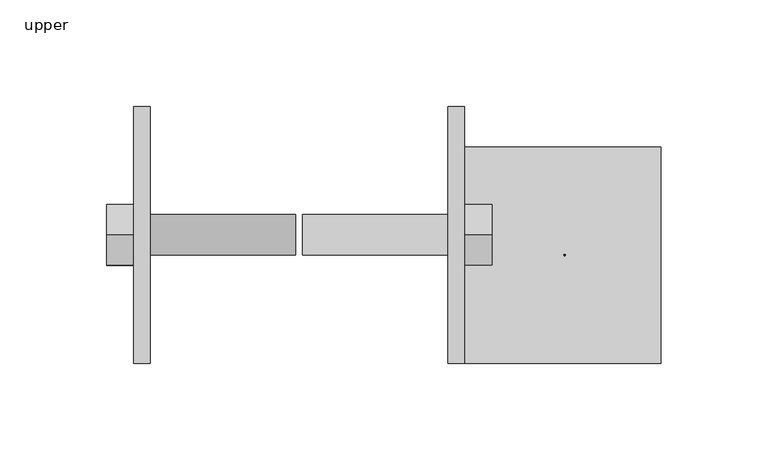
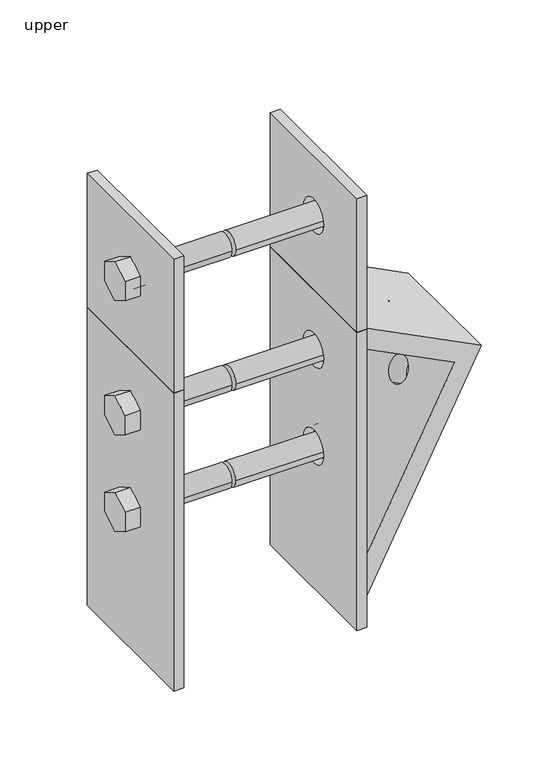
"""IFC4 building model written with IfcOpenShell, lengths in millimetres: fastener geometry, 060523 - W_P_C - Fastenings - Column Base & Top with X Bracing - Custom : upper."""

from ifc_helpers import new_model, si_unit, point, frame, frame_2d, origin, place, context, project, spatial, polyline, circle_curve, trimmed, segment, composite_curve, outline, extrude, source, transform, mapped, element, save
from ifc_brep_helpers import plane_surface, revolved_surface, advanced_brep


def upper_50ad7738(model_context):
    return source(origin(), model_context, "Body", "SolidModel", [
        advanced_brep(
        [(-77.7875, 60.325, 261.9375), (-77.7875, -52.3875, 261.9375), (-77.7875, -60.325, 261.9375), (-69.85, -60.325, 261.9375), (-69.85, 60.325, 261.9375), (-77.7875, 60.325, 7.9375), (-77.7875, -52.3875, 7.9375), (-77.7875, -60.325, 7.9375), (-77.7875, -13.890625, 211.1375), (-77.7875, 13.890625, 211.1375), (-77.7875, -13.890625, 128.5875), (-77.7875, 13.890625, 128.5875), (-69.85, 60.325, 7.9375), (-69.85, -60.325, 7.9375), (-69.85, 13.890625, 211.1375), (-69.85, -13.890625, 211.1375), (-69.85, 13.890625, 128.5875), (-69.85, -13.890625, 128.5875)],
        [
            (0, 1),
            (1, 2),
            (2, 3),
            (3, 4),
            (4, 0),
            (0, 5),
            (5, 6),
            (6, 7),
            (7, 2),
            (8, 9, circle_curve(frame((-77.7875, 0.0, 211.1375), z_axis=(1.0, 0.0, 0.0), x_axis=(0.0, -1.0, 0.0)), 13.890625)),
            (9, 8, circle_curve(frame((-77.7875, 0.0, 211.1375), z_axis=(1.0, 0.0, 0.0), x_axis=(0.0, -1.0, 0.0)), 13.890625)),
            (10, 11, circle_curve(frame((-77.7875, 0.0, 128.5875), z_axis=(1.0, 0.0, 0.0), x_axis=(0.0, -1.0, 0.0)), 13.890625)),
            (11, 10, circle_curve(frame((-77.7875, 0.0, 128.5875), z_axis=(1.0, 0.0, 0.0), x_axis=(0.0, -1.0, 0.0)), 13.890625)),
            (4, 12),
            (12, 5),
            (7, 13),
            (13, 3),
            (14, 9),
            (8, 15),
            (15, 14, circle_curve(frame((-69.85, 0.0, 211.1375), z_axis=(1.0, 0.0, 0.0), x_axis=(0.0, -1.0, 0.0)), 13.890625)),
            (14, 15, circle_curve(frame((-69.85, 0.0, 211.1375), z_axis=(1.0, 0.0, 0.0), x_axis=(0.0, -1.0, 0.0)), 13.890625)),
            (16, 11),
            (10, 17),
            (17, 16, circle_curve(frame((-69.85, 0.0, 128.5875), z_axis=(1.0, 0.0, 0.0), x_axis=(0.0, -1.0, 0.0)), 13.890625)),
            (16, 17, circle_curve(frame((-69.85, 0.0, 128.5875), z_axis=(1.0, 0.0, 0.0), x_axis=(0.0, -1.0, 0.0)), 13.890625)),
            (13, 12),
        ],
        [
            plane_surface(frame((-77.7875, -60.325, 261.9375), z_axis=(0.0, 0.0, 1.0), x_axis=(1.0, 0.0, 0.0))),
            plane_surface(frame((-77.7875, 60.325, 261.9375), z_axis=(-1.0, 0.0, 0.0), x_axis=(0.0, 1.0, 0.0))),
            plane_surface(frame((-77.7875, 60.325, 261.9375), z_axis=(0.0, 1.0, 0.0), x_axis=(1.0, 0.0, 0.0))),
            plane_surface(frame((-77.7875, -60.325, 7.9375), z_axis=(0.0, -1.0, 0.0), x_axis=(1.0, 0.0, 0.0))),
            revolved_surface(polyline([(-77.7875, -13.890625, 211.1375), (-69.85, -13.890625, 211.1375)]), (-69.85, 0.0, 211.1375), (-1.0, 0.0, 0.0)),
            revolved_surface(polyline([(-77.7875, -13.890625, 128.5875), (-69.85, -13.890625, 128.5875)]), (-69.85, 0.0, 128.5875), (-1.0, 0.0, 0.0)),
            plane_surface(frame((-69.85, 60.325, 261.9375), z_axis=(1.0, 0.0, 0.0), x_axis=(0.0, -1.0, 0.0))),
            plane_surface(frame((-77.7875, 60.325, 7.9375), z_axis=(0.0, 0.0, -1.0), x_axis=(1.0, 0.0, 0.0))),
        ],
        [
            (0, [[1, 2, 3, 4, 5]]),
            (1, [[-2, -1, 6, 7, 8, 9], [10, 11], [12, 13]]),
            (2, [[-6, -5, 14, 15]]),
            (3, [[-9, 16, 17, -3]]),
            (4, [[18, -10, 19, 20]]),
            (4, [[-18, 21, -19, -11]]),
            (5, [[22, -12, 23, 24]]),
            (5, [[-22, 25, -23, -13]]),
            (6, [[-17, 26, -14, -4], [-20, -21], [-24, -25]]),
            (7, [[-8, -7, -15, -26, -16]]),
        ],
    ),
        extrude(outline(polyline([(14.2875, 219.386392), (14.2875, 202.888608), (0.0, 194.6397161), (-14.2875, 202.888608), (-14.2875, 219.386392), (0.0, 227.6352839), (14.2875, 219.386392)])), frame((-90.4875, 0.0, 0.0), z_axis=(1.0, 0.0, 0.0), x_axis=(0.0, 1.0, 0.0)), (0.0, 0.0, 1.0), 12.7),
        extrude(outline(composite_curve([segment(trimmed(circle_curve(frame_2d((0.0, 211.1375)), 9.525), [point((9.525, 211.1375))], [point((-9.525, 211.1375))], False, "CARTESIAN"), True, "CONTINUOUS"), segment(trimmed(circle_curve(frame_2d((0.0, 211.1375)), 9.525), [point((-9.525, 211.1375))], [point((9.525, 211.1375))], False, "CARTESIAN"), True, "CONTINUOUS")], self_intersect=False)), frame((-77.7875, 0.0, 0.0), z_axis=(1.0, 0.0, 0.0), x_axis=(0.0, 1.0, 0.0)), (0.0, 0.0, 1.0), 76.2),
        extrude(outline(polyline([(14.2875, 136.836392), (14.2875, 120.338608), (0.0, 112.0897161), (-14.2875, 120.338608), (-14.2875, 136.836392), (0.0, 145.0852839), (14.2875, 136.836392)])), frame((-90.4875, 0.0, 0.0), z_axis=(1.0, 0.0, 0.0), x_axis=(0.0, 1.0, 0.0)), (0.0, 0.0, 1.0), 12.7),
        extrude(outline(composite_curve([segment(trimmed(circle_curve(frame_2d((0.0, 128.5875)), 9.525), [point((9.525, 128.5875))], [point((-9.525, 128.5875))], False, "CARTESIAN"), True, "CONTINUOUS"), segment(trimmed(circle_curve(frame_2d((0.0, 128.5875)), 9.525), [point((-9.525, 128.5875))], [point((9.525, 128.5875))], False, "CARTESIAN"), True, "CONTINUOUS")], self_intersect=False)), frame((-77.7875, 0.0, 0.0), z_axis=(1.0, 0.0, 0.0), x_axis=(0.0, 1.0, 0.0)), (0.0, 0.0, 1.0), 76.2),
        extrude(outline(polyline([(14.2875, 219.386392), (14.2875, 202.888608), (0.0, 194.6397161), (-14.2875, 202.888608), (-14.2875, 219.386392), (0.0, 227.6352839), (14.2875, 219.386392)])), frame((-90.4875, 0.0, 0.0), z_axis=(1.0, 0.0, 0.0), x_axis=(0.0, 1.0, 0.0)), (0.0, 0.0, 1.0), 12.7),
        extrude(outline(composite_curve([segment(trimmed(circle_curve(frame_2d((0.0, 211.1375)), 9.525), [point((9.525, 211.1375))], [point((-9.525, 211.1375))], False, "CARTESIAN"), True, "CONTINUOUS"), segment(trimmed(circle_curve(frame_2d((0.0, 211.1375)), 9.525), [point((-9.525, 211.1375))], [point((9.525, 211.1375))], False, "CARTESIAN"), True, "CONTINUOUS")], self_intersect=False)), frame((-77.7875, 0.0, 0.0), z_axis=(1.0, 0.0, 0.0), x_axis=(0.0, 1.0, 0.0)), (0.0, 0.0, 1.0), 76.2),
        advanced_brep(
        [(77.7875, 60.325, 261.9375), (69.85, 60.325, 261.9375), (69.85, -60.325, 261.9375), (77.7875, -60.325, 261.9375), (77.7875, -52.3875, 261.9375), (77.7875, -60.325, 7.9375), (77.7875, -52.3875, 7.9375), (77.7875, 60.325, 7.9375), (77.7875, -13.890625, 211.1375), (77.7875, 13.890625, 211.1375), (77.7875, -13.890625, 128.5875), (77.7875, 13.890625, 128.5875), (69.85, 60.325, 7.9375), (69.85, -60.325, 7.9375), (69.85, 13.890625, 211.1375), (69.85, -13.890625, 211.1375), (69.85, 13.890625, 128.5875), (69.85, -13.890625, 128.5875)],
        [
            (0, 1),
            (1, 2),
            (2, 3),
            (3, 4),
            (4, 0),
            (3, 5),
            (5, 6),
            (6, 7),
            (7, 0),
            (8, 9, circle_curve(frame((77.7875, 0.0, 211.1375), z_axis=(-1.0, 0.0, 0.0), x_axis=(0.0, -1.0, 0.0)), 13.890625)),
            (9, 8, circle_curve(frame((77.7875, 0.0, 211.1375), z_axis=(-1.0, 0.0, 0.0), x_axis=(0.0, -1.0, 0.0)), 13.890625)),
            (10, 11, circle_curve(frame((77.7875, 0.0, 128.5875), z_axis=(-1.0, 0.0, 0.0), x_axis=(0.0, -1.0, 0.0)), 13.890625)),
            (11, 10, circle_curve(frame((77.7875, 0.0, 128.5875), z_axis=(-1.0, 0.0, 0.0), x_axis=(0.0, -1.0, 0.0)), 13.890625)),
            (7, 12),
            (12, 1),
            (2, 13),
            (13, 5),
            (14, 15, circle_curve(frame((69.85, 0.0, 211.1375), z_axis=(-1.0, 0.0, 0.0), x_axis=(0.0, -1.0, 0.0)), 13.890625)),
            (15, 8),
            (9, 14),
            (15, 14, circle_curve(frame((69.85, 0.0, 211.1375), z_axis=(-1.0, 0.0, 0.0), x_axis=(0.0, -1.0, 0.0)), 13.890625)),
            (16, 17, circle_curve(frame((69.85, 0.0, 128.5875), z_axis=(-1.0, 0.0, 0.0), x_axis=(0.0, -1.0, 0.0)), 13.890625)),
            (17, 10),
            (11, 16),
            (17, 16, circle_curve(frame((69.85, 0.0, 128.5875), z_axis=(-1.0, 0.0, 0.0), x_axis=(0.0, -1.0, 0.0)), 13.890625)),
            (12, 13),
        ],
        [
            plane_surface(frame((77.7875, -60.325, 261.9375), z_axis=(0.0, 0.0, 1.0), x_axis=(-1.0, 0.0, 0.0))),
            plane_surface(frame((77.7875, 60.325, 261.9375), z_axis=(1.0, 0.0, 0.0), x_axis=(0.0, 1.0, 0.0))),
            plane_surface(frame((77.7875, 60.325, 261.9375), z_axis=(0.0, 1.0, 0.0), x_axis=(-1.0, 0.0, 0.0))),
            plane_surface(frame((77.7875, -60.325, 7.9375), z_axis=(0.0, -1.0, 0.0), x_axis=(-1.0, 0.0, 0.0))),
            revolved_surface(polyline([(77.7875, -13.890625, 211.1375), (69.85, -13.890625, 211.1375)]), (69.85, 0.0, 211.1375), (1.0, 0.0, 0.0)),
            revolved_surface(polyline([(77.7875, -13.890625, 128.5875), (69.85, -13.890625, 128.5875)]), (69.85, 0.0, 128.5875), (1.0, 0.0, 0.0)),
            plane_surface(frame((69.85, 60.325, 261.9375), z_axis=(-1.0, 0.0, 0.0), x_axis=(0.0, -1.0, 0.0))),
            plane_surface(frame((77.7875, 60.325, 7.9375), z_axis=(0.0, 0.0, -1.0), x_axis=(-1.0, 0.0, 0.0))),
        ],
        [
            (0, [[1, 2, 3, 4, 5]]),
            (1, [[6, 7, 8, 9, -5, -4], [10, 11], [12, 13]]),
            (2, [[14, 15, -1, -9]]),
            (3, [[-3, 16, 17, -6]]),
            (4, [[18, 19, -11, 20]]),
            (4, [[-10, -19, 21, -20]]),
            (5, [[22, 23, -13, 24]]),
            (5, [[-12, -23, 25, -24]]),
            (6, [[-2, -15, 26, -16], [-21, -18], [-25, -22]]),
            (7, [[-17, -26, -14, -8, -7]]),
        ],
    ),
        extrude(outline(polyline([(14.2875, 219.386392), (14.2875, 202.888608), (0.0, 194.6397161), (-14.2875, 202.888608), (-14.2875, 219.386392), (0.0, 227.6352839), (14.2875, 219.386392)])), frame((77.7875, 0.0, 0.0), z_axis=(1.0, 0.0, 0.0), x_axis=(0.0, 1.0, 0.0)), (0.0, 0.0, 1.0), 12.7),
        extrude(outline(composite_curve([segment(trimmed(circle_curve(frame_2d((0.0, 211.1375)), 9.525), [point((9.525, 211.1375))], [point((-9.525, 211.1375))], False, "CARTESIAN"), True, "CONTINUOUS"), segment(trimmed(circle_curve(frame_2d((0.0, 211.1375)), 9.525), [point((-9.525, 211.1375))], [point((9.525, 211.1375))], False, "CARTESIAN"), True, "CONTINUOUS")], self_intersect=False)), frame((1.5875, 0.0, 0.0), z_axis=(1.0, 0.0, 0.0), x_axis=(0.0, 1.0, 0.0)), (0.0, 0.0, 1.0), 76.2),
        extrude(outline(polyline([(14.2875, 136.836392), (14.2875, 120.338608), (0.0, 112.0897161), (-14.2875, 120.338608), (-14.2875, 136.836392), (0.0, 145.0852839), (14.2875, 136.836392)])), frame((77.7875, 0.0, 0.0), z_axis=(1.0, 0.0, 0.0), x_axis=(0.0, 1.0, 0.0)), (0.0, 0.0, 1.0), 12.7),
        extrude(outline(composite_curve([segment(trimmed(circle_curve(frame_2d((0.0, 128.5875)), 9.525), [point((9.525, 128.5875))], [point((-9.525, 128.5875))], False, "CARTESIAN"), True, "CONTINUOUS"), segment(trimmed(circle_curve(frame_2d((0.0, 128.5875)), 9.525), [point((-9.525, 128.5875))], [point((9.525, 128.5875))], False, "CARTESIAN"), True, "CONTINUOUS")], self_intersect=False)), frame((1.5875, 0.0, 0.0), z_axis=(1.0, 0.0, 0.0), x_axis=(0.0, 1.0, 0.0)), (0.0, 0.0, 1.0), 76.2),
        extrude(outline(polyline([(14.2875, 219.386392), (14.2875, 202.888608), (0.0, 194.6397161), (-14.2875, 202.888608), (-14.2875, 219.386392), (0.0, 227.6352839), (14.2875, 219.386392)])), frame((77.7875, 0.0, 0.0), z_axis=(1.0, 0.0, 0.0), x_axis=(0.0, 1.0, 0.0)), (0.0, 0.0, 1.0), 12.7),
        extrude(outline(composite_curve([segment(trimmed(circle_curve(frame_2d((0.0, 211.1375)), 9.525), [point((9.525, 211.1375))], [point((-9.525, 211.1375))], False, "CARTESIAN"), True, "CONTINUOUS"), segment(trimmed(circle_curve(frame_2d((0.0, 211.1375)), 9.525), [point((-9.525, 211.1375))], [point((9.525, 211.1375))], False, "CARTESIAN"), True, "CONTINUOUS")], self_intersect=False)), frame((1.5875, 0.0, 0.0), z_axis=(1.0, 0.0, 0.0), x_axis=(0.0, 1.0, 0.0)), (0.0, 0.0, 1.0), 76.2),
        advanced_brep(
        [(-77.7875, -60.325, 376.2375), (-77.7875, 60.325, 376.2375), (-77.7875, 60.325, 261.9375), (-77.7875, 52.3875, 261.9375), (-77.7875, -60.325, 261.9375), (-77.7875, -13.890625, 325.4375), (-77.7875, 13.890625, 325.4375), (-69.85, -60.325, 376.2375), (-69.85, 60.325, 376.2375), (-69.85, 60.325, 261.9375), (-69.85, -60.325, 261.9375), (-69.85, 13.890625, 325.4375), (-69.85, -13.890625, 325.4375)],
        [
            (0, 1),
            (1, 2),
            (2, 3),
            (3, 4),
            (4, 0),
            (5, 6, circle_curve(frame((-77.7875, 0.0, 325.4375), z_axis=(1.0, 0.0, 0.0), x_axis=(0.0, -1.0, 0.0)), 13.890625)),
            (6, 5, circle_curve(frame((-77.7875, 0.0, 325.4375), z_axis=(1.0, 0.0, 0.0), x_axis=(0.0, -1.0, 0.0)), 13.890625)),
            (0, 7),
            (7, 8),
            (8, 1),
            (8, 9),
            (9, 2),
            (4, 10),
            (10, 7),
            (11, 6),
            (5, 12),
            (12, 11, circle_curve(frame((-69.85, 0.0, 325.4375), z_axis=(1.0, 0.0, 0.0), x_axis=(0.0, -1.0, 0.0)), 13.890625)),
            (11, 12, circle_curve(frame((-69.85, 0.0, 325.4375), z_axis=(1.0, 0.0, 0.0), x_axis=(0.0, -1.0, 0.0)), 13.890625)),
            (10, 9),
        ],
        [
            plane_surface(frame((-77.7875, 60.325, 376.2375), z_axis=(-1.0, 0.0, 0.0), x_axis=(0.0, 1.0, 0.0))),
            plane_surface(frame((-77.7875, -60.325, 376.2375), z_axis=(0.0, 0.0, 1.0), x_axis=(1.0, 0.0, 0.0))),
            plane_surface(frame((-77.7875, 60.325, 376.2375), z_axis=(0.0, 1.0, 0.0), x_axis=(1.0, 0.0, 0.0))),
            plane_surface(frame((-77.7875, -60.325, 261.9375), z_axis=(0.0, -1.0, 0.0), x_axis=(1.0, 0.0, 0.0))),
            revolved_surface(polyline([(-77.7875, -13.890625, 325.4375), (-69.85, -13.890625, 325.4375)]), (-69.85, 0.0, 325.4375), (-1.0, 0.0, 0.0)),
            plane_surface(frame((-69.85, 60.325, 376.2375), z_axis=(1.0, 0.0, 0.0), x_axis=(0.0, -1.0, 0.0))),
            plane_surface(frame((-77.7875, 60.325, 261.9375), z_axis=(0.0, 0.0, -1.0), x_axis=(1.0, 0.0, 0.0))),
        ],
        [
            (0, [[1, 2, 3, 4, 5], [6, 7]]),
            (1, [[-1, 8, 9, 10]]),
            (2, [[-2, -10, 11, 12]]),
            (3, [[-5, 13, 14, -8]]),
            (4, [[15, -6, 16, 17]]),
            (4, [[-15, 18, -16, -7]]),
            (5, [[-14, 19, -11, -9], [-17, -18]]),
            (6, [[-4, -3, -12, -19, -13]]),
        ],
    ),
        extrude(outline(polyline([(14.2875, 333.686392), (14.2875, 317.188608), (0.0, 308.9397161), (-14.2875, 317.188608), (-14.2875, 333.686392), (0.0, 341.9352839), (14.2875, 333.686392)])), frame((-90.4875, 0.0, 0.0), z_axis=(1.0, 0.0, 0.0), x_axis=(0.0, 1.0, 0.0)), (0.0, 0.0, 1.0), 12.7),
        extrude(outline(composite_curve([segment(trimmed(circle_curve(frame_2d((0.0, 325.4375)), 9.525), [point((9.525, 325.4375))], [point((-9.525, 325.4375))], False, "CARTESIAN"), True, "CONTINUOUS"), segment(trimmed(circle_curve(frame_2d((0.0, 325.4375)), 9.525), [point((-9.525, 325.4375))], [point((9.525, 325.4375))], False, "CARTESIAN"), True, "CONTINUOUS")], self_intersect=False)), frame((-77.7875, 0.0, 0.0), z_axis=(1.0, 0.0, 0.0), x_axis=(0.0, 1.0, 0.0)), (0.0, 0.0, 1.0), 76.2),
        advanced_brep(
        [(77.7875, -60.325, 376.2375), (77.7875, -60.325, 261.9375), (77.7875, 52.3875, 261.9375), (77.7875, 60.325, 261.9375), (77.7875, 60.325, 376.2375), (77.7875, -13.890625, 325.4375), (77.7875, 13.890625, 325.4375), (69.85, 60.325, 376.2375), (69.85, -60.325, 376.2375), (69.85, 60.325, 261.9375), (69.85, -60.325, 261.9375), (69.85, 13.890625, 325.4375), (69.85, -13.890625, 325.4375)],
        [
            (0, 1),
            (1, 2),
            (2, 3),
            (3, 4),
            (4, 0),
            (5, 6, circle_curve(frame((77.7875, 0.0, 325.4375), z_axis=(-1.0, 0.0, 0.0), x_axis=(0.0, -1.0, 0.0)), 13.890625)),
            (6, 5, circle_curve(frame((77.7875, 0.0, 325.4375), z_axis=(-1.0, 0.0, 0.0), x_axis=(0.0, -1.0, 0.0)), 13.890625)),
            (4, 7),
            (7, 8),
            (8, 0),
            (3, 9),
            (9, 7),
            (8, 10),
            (10, 1),
            (11, 12, circle_curve(frame((69.85, 0.0, 325.4375), z_axis=(-1.0, 0.0, 0.0), x_axis=(0.0, -1.0, 0.0)), 13.890625)),
            (12, 5),
            (6, 11),
            (12, 11, circle_curve(frame((69.85, 0.0, 325.4375), z_axis=(-1.0, 0.0, 0.0), x_axis=(0.0, -1.0, 0.0)), 13.890625)),
            (9, 10),
        ],
        [
            plane_surface(frame((77.7875, 60.325, 376.2375), z_axis=(1.0, 0.0, 0.0), x_axis=(0.0, 1.0, 0.0))),
            plane_surface(frame((77.7875, -60.325, 376.2375), z_axis=(0.0, 0.0, 1.0), x_axis=(-1.0, 0.0, 0.0))),
            plane_surface(frame((77.7875, 60.325, 376.2375), z_axis=(0.0, 1.0, 0.0), x_axis=(-1.0, 0.0, 0.0))),
            plane_surface(frame((77.7875, -60.325, 261.9375), z_axis=(0.0, -1.0, 0.0), x_axis=(-1.0, 0.0, 0.0))),
            revolved_surface(polyline([(77.7875, -13.890625, 325.4375), (69.85, -13.890625, 325.4375)]), (69.85, 0.0, 325.4375), (1.0, 0.0, 0.0)),
            plane_surface(frame((69.85, 60.325, 376.2375), z_axis=(-1.0, 0.0, 0.0), x_axis=(0.0, -1.0, 0.0))),
            plane_surface(frame((77.7875, 60.325, 261.9375), z_axis=(0.0, 0.0, -1.0), x_axis=(-1.0, 0.0, 0.0))),
        ],
        [
            (0, [[1, 2, 3, 4, 5], [6, 7]]),
            (1, [[8, 9, 10, -5]]),
            (2, [[11, 12, -8, -4]]),
            (3, [[-10, 13, 14, -1]]),
            (4, [[15, 16, -7, 17]]),
            (4, [[-6, -16, 18, -17]]),
            (5, [[-9, -12, 19, -13], [-18, -15]]),
            (6, [[-14, -19, -11, -3, -2]]),
        ],
    ),
        extrude(outline(polyline([(14.2875, 333.686392), (14.2875, 317.188608), (0.0, 308.9397161), (-14.2875, 317.188608), (-14.2875, 333.686392), (0.0, 341.9352839), (14.2875, 333.686392)])), frame((77.7875, 0.0, 0.0), z_axis=(1.0, 0.0, 0.0), x_axis=(0.0, 1.0, 0.0)), (0.0, 0.0, 1.0), 12.7),
        extrude(outline(composite_curve([segment(trimmed(circle_curve(frame_2d((0.0, 325.4375)), 9.525), [point((9.525, 325.4375))], [point((-9.525, 325.4375))], False, "CARTESIAN"), True, "CONTINUOUS"), segment(trimmed(circle_curve(frame_2d((0.0, 325.4375)), 9.525), [point((-9.525, 325.4375))], [point((9.525, 325.4375))], False, "CARTESIAN"), True, "CONTINUOUS")], self_intersect=False)), frame((1.5875, 0.0, 0.0), z_axis=(1.0, 0.0, 0.0), x_axis=(0.0, 1.0, 0.0)), (0.0, 0.0, 1.0), 76.2),
        advanced_brep(
        [(170.0383695, 41.275, 215.9775257), (77.7875, 41.275, 34.925), (77.7875, 41.275, 69.8926921), (148.6865418, 41.275, 209.0398963), (77.7875, 41.275, 245.1647625), (77.7875, 41.275, 262.9816915), (170.0383695, -60.325, 215.9775257), (77.7875, -60.325, 262.9816915), (77.7875, -60.325, 245.1647625), (148.6865418, -60.325, 209.0398963), (77.7875, -60.325, 69.8926921), (77.7875, -60.325, 34.925), (125.1288563, -9.525, 238.8600656), (124.4216199, -9.525, 239.2204206), (117.2145207, -9.525, 225.075692), (117.9217571, -9.525, 224.7153371), (137.6957155, -9.525, 187.4691853), (127.9661316, -9.525, 168.3738017), (142.1108602, -9.525, 161.1667025), (151.8404441, -9.525, 180.2620861)],
        [
            (0, 1),
            (1, 2),
            (2, 3),
            (3, 4),
            (4, 5),
            (5, 0),
            (6, 7),
            (7, 8),
            (8, 9),
            (9, 10),
            (10, 11),
            (11, 6),
            (5, 7),
            (6, 0),
            (12, 13, circle_curve(frame((124.7752381, -9.525, 239.0402431), z_axis=(-0.45399049973954897, 0.0, -0.8910065241883668), x_axis=(-0.8910065241883668, 0.0, 0.45399049973954897)), 0.396875)),
            (13, 12, circle_curve(frame((124.7752381, -9.525, 239.0402431), z_axis=(-0.45399049973954897, 0.0, -0.8910065241883668), x_axis=(-0.8910065241883668, 0.0, 0.45399049973954897)), 0.396875)),
            (4, 8),
            (3, 9),
            (14, 15, circle_curve(frame((117.5681389, -9.525, 224.8955145), z_axis=(0.45399049973954897, 0.0, 0.8910065241883668), x_axis=(-0.8910065241883668, 0.0, 0.45399049973954897)), 0.396875)),
            (15, 14, circle_curve(frame((117.5681389, -9.525, 224.8955145), z_axis=(0.45399049973954897, 0.0, 0.8910065241883668), x_axis=(-0.8910065241883668, 0.0, 0.45399049973954897)), 0.396875)),
            (2, 10),
            (16, 17, circle_curve(frame((132.8309236, -9.525, 177.9214935), z_axis=(0.8910065241883661, 0.0, -0.4539904997395502), x_axis=(0.4539904997395502, 0.0, 0.8910065241883661)), 10.715625)),
            (17, 16, circle_curve(frame((132.8309236, -9.525, 177.9214935), z_axis=(0.8910065241883661, 0.0, -0.4539904997395502), x_axis=(0.4539904997395502, 0.0, 0.8910065241883661)), 10.715625)),
            (1, 11),
            (18, 19, circle_curve(frame((146.9756522, -9.525, 170.7143943), z_axis=(-0.8910065241883661, 0.0, 0.4539904997395502), x_axis=(0.4539904997395502, 0.0, 0.8910065241883661)), 10.715625)),
            (19, 18, circle_curve(frame((146.9756522, -9.525, 170.7143943), z_axis=(-0.8910065241883661, 0.0, 0.4539904997395502), x_axis=(0.4539904997395502, 0.0, 0.8910065241883661)), 10.715625)),
            (13, 14),
            (15, 12),
            (19, 16),
            (17, 18),
        ],
        [
            plane_surface(frame((77.7875, 41.275, 262.9816915), z_axis=(0.0, 1.0, 0.0), x_axis=(-0.8910065241883668, 0.0, 0.45399049973954897))),
            plane_surface(frame((77.7875, -60.325, 262.9816915), z_axis=(0.0, -1.0, 0.0), x_axis=(0.8910065241883668, 0.0, -0.45399049973954897))),
            plane_surface(frame((170.0383695, 41.275, 215.9775257), z_axis=(0.45399049973954897, 0.0, 0.8910065241883668), x_axis=(0.0, -1.0, 0.0))),
            plane_surface(frame((77.7875, 41.275, 262.9816915), z_axis=(-1.0, 0.0, 0.0), x_axis=(0.0, -1.0, 0.0))),
            plane_surface(frame((77.7875, 41.275, 245.1647625), z_axis=(-0.4539904997395488, 0.0, -0.8910065241883668), x_axis=(0.0, -1.0, 0.0))),
            plane_surface(frame((148.6865418, 41.275, 209.0398963), z_axis=(-0.8910065241883659, 0.0, 0.45399049973955063), x_axis=(0.0, -1.0, 0.0))),
            plane_surface(frame((77.7875, 41.275, 69.8926921), z_axis=(-1.0, 0.0, 0.0), x_axis=(0.0, -1.0, 0.0))),
            plane_surface(frame((77.7875, 41.275, 34.925), z_axis=(0.8910065241883661, 0.0, -0.4539904997395502), x_axis=(0.0, -1.0, 0.0))),
            revolved_surface(polyline([(117.21452068738647, -9.525, 225.0756919787313), (124.42161989691586, -9.525, 239.22042060157148)]), (124.7752381, -9.525, 239.0402431), (-0.45399049973954897, 0.0, -0.8910065241883668)),
            revolved_surface(polyline([(137.69571550343758, -9.525, 187.4691853067466), (151.84044414877164, -9.525, 180.26208608575598)]), (146.9756522, -9.525, 170.7143943), (-0.8910065241883661, 0.0, 0.4539904997395502)),
        ],
        [
            (0, [[1, 2, 3, 4, 5, 6]]),
            (1, [[7, 8, 9, 10, 11, 12]]),
            (2, [[13, -7, 14, -6], [15, 16]]),
            (3, [[17, -8, -13, -5]]),
            (4, [[18, -9, -17, -4], [19, 20]]),
            (5, [[21, -10, -18, -3], [22, 23]]),
            (6, [[24, -11, -21, -2]]),
            (7, [[-14, -12, -24, -1], [25, 26]]),
            (8, [[-16, 27, -20, 28]]),
            (8, [[-19, -27, -15, -28]]),
            (9, [[-26, 29, -23, 30]]),
            (9, [[-22, -29, -25, -30]]),
        ],
    ),
    ])


if __name__ == "__main__":
    model = new_model("IFC4")
    model_context = context("Model", 3, world=origin())
    ifc_project = project(units=[si_unit("LENGTHUNIT", "METRE", prefix="MILLI")], contexts=[model_context])
    site = spatial("IfcSite", under=ifc_project)
    building = spatial("IfcBuilding", under=site)
    placement = place(None, origin())
    upper_shape = upper_50ad7738(model_context)
    element("IfcFastener", 1, ObjectType="060523 - W_P_C - Fastenings - Column Base & Top with X Bracing - Custom : upper", at=placement, inside=building, context=model_context, shape_type="MappedRepresentation", body=[
        mapped(upper_shape, transform((0.0, 0.0, 0.0), x_axis=(1.0, 0.0, 0.0), y_axis=(0.0, 1.0, 0.0), z_axis=(0.0, 0.0, 1.0))),
    ])
    save(model, "model.ifc")

# Revit data of these elements
# Type "060523 - W_P_C - Fastenings - Column Base & Top with X Bracing - Custom : upper"
#   Width - Top = 0' - 5 1/2"
#   Top/Bottom Plate Thickness = 0' - 0 5/16"
#   Top/Bottom Plate - Width = 0' - 7 1/2"
#   Rod Radius = 0' - 0 3/8"
#   Rod Length [instance default] = 1' - 0"
#   Plate Thickness = 0' - 0 5/16"
#   Offset - Upper Plate 2 = 0' - 0"
#   Height of Plate = 0' - 10"
#   Width - Bottom = 0' - 5 1/2"
#   Plate Width = 0' - 4 3/4"
#   Bracket Width = 0' - 4"
#   Bracket Thickness = 0' - 0 5/8"
#   Bracket Offset in X = 0' - 3 1/16"
#   Bracket Offset in Y = 0' - 0"
#   Bracket Offset = 0' - 1 3/8"
#   Bracket Leg = 0' - 8"
#   Bracket Hole Radius - Up = 0' - 0 1/64"
#   Bracket Hole Radius - Down = 0' - 0 27/64"
#   Bracket Hole Offset = 0' - 2"
#   Beam Width = 0' - 7 3/8"
#   Angle 2 = 63.00°
#   Angle 1 = 153.00°
#   Top Plate Visible = no
#   Rod Visibility = no
#   Plate Visibility - Upper Right 2 = no
#   Plate Visibility - Upper Right 1 = yes
#   Plate Visibility - Upper Left 2 = no
#   Plate Visibility - Upper Left 1 = yes
#   Plate Visibility - Lower Right 2 = no
#   Plate Visibility - Lower Right 1 = yes
#   Plate Visibility - Lower Left 2 = no
#   Plate Visibility - Lower Left 1 = yes
#   Bracket Visibility = yes
#   Bottom Plate Visible = no
#   Upper Plates - 2 = element 1925096
#   Upper Plates - 1 = element 1925090
#   Rod Material = 3/4" STEEL (RAW) ROD (THREADED AT ENDS) - W/ TURNBUCKLE
#   Lower Plates = element 1925094
#   Bracket Material = 5/8" STEEL ANGLE (RAW STEEL)
#   URL = ""
# Element 1 (IfcFastener, "060523 - W_P_C - Fastenings - Column Base & Top with X Bracing - Custom : upper")
#   Rod Length = 11' - 3"
#   Materials on its faces: "3/4\" LAG BOLT (THRU BOLT IF PLATE ON OPP. SIDE OF STRUCT MEMBER)", "5/16\" STEEL PLATE (RAW STEEL)", "5/8\" STEEL ANGLE (RAW STEEL)"
# Materials
#   "3/4\" STEEL (RAW) ROD (THREADED AT ENDS) - W/ TURNBUCKLE": class "Generic", colour RGB 120 120 120, transparency 0, Cost = 0
#   "5/8\" STEEL ANGLE (RAW STEEL)": class "Generic", colour RGB 195 195 195, transparency 0, Cost = 0
#   "3/4\" LAG BOLT (THRU BOLT IF PLATE ON OPP. SIDE OF STRUCT MEMBER)": class "Generic", colour RGB 120 120 120, transparency 0, Cost = 0
#   "5/16\" STEEL PLATE (RAW STEEL)": class "Generic", colour RGB 232 232 232, transparency 0, Cost = 0
